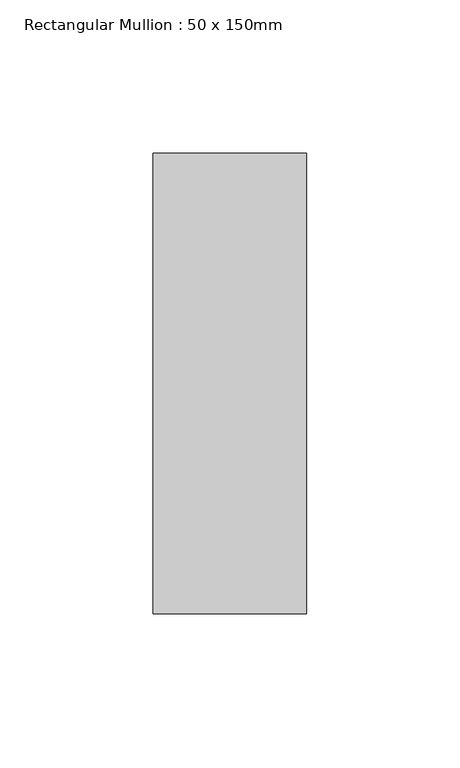
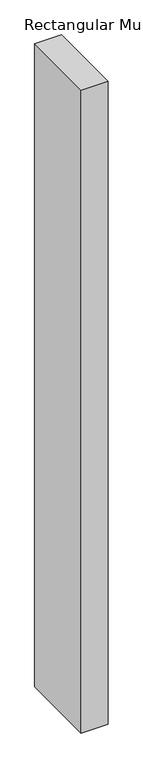
"""IFC4 building model written with IfcOpenShell, lengths in millimetres: member geometry, Rectangular Mullion : 50 x 150mm."""

from ifc_helpers import new_model, si_unit, frame, origin, place, context, project, spatial, polyline, outline, extrude, source, transform, mapped, element, save


def rectangular_mullion_50_x_150mm_673792d4(model_context):
    return source(origin(), model_context, "Body", "SweptSolid", [
        extrude(outline(polyline([(0.0, 75.0), (0.0, -75.0), (-50.0, -75.0), (-50.0, 75.0), (0.0, 75.0)])), frame((0.0, 0.0, -1264.9999999), z_axis=(0.0, 0.0, 1.0), x_axis=(1.0, 0.0, 0.0)), (0.0, 0.0, 1.0), 1264.9999999),
    ])


if __name__ == "__main__":
    model = new_model("IFC4")
    model_context = context("Model", 3, world=origin())
    ifc_project = project(units=[si_unit("LENGTHUNIT", "METRE", prefix="MILLI")], contexts=[model_context])
    site = spatial("IfcSite", under=ifc_project)
    building = spatial("IfcBuilding", under=site)
    placement = place(None, origin())
    rectangular_mullion_50_x_150mm_shape = rectangular_mullion_50_x_150mm_673792d4(model_context)
    element("IfcMember", 1, ObjectType="Rectangular Mullion : 50 x 150mm", at=placement, inside=building, context=model_context, shape_type="MappedRepresentation", body=[
        mapped(rectangular_mullion_50_x_150mm_shape, transform((0.0, 0.0, 0.0), x_axis=(1.0, 0.0, 0.0), y_axis=(0.0, 1.0, 0.0), z_axis=(0.0, 0.0, 1.0))),
    ])
    save(model, "model.ifc")

# Revit data of these elements
# Type "Rectangular Mullion : 50 x 150mm"
#   built-in parameter 1007304 = 0.492126 (stored number, unit not read)
#   built-in parameter 1007301 = 0.082021 (stored number, unit not read)
#   built-in parameter 1007300 = 0.082021 (stored number, unit not read)
# Element 1 (IfcMember, "Rectangular Mullion : 50 x 150mm")
#   Materials on its faces: "Aluminium"
# Materials
#   "Aluminium": class "Metal", colour RGB 247 247 247, transparency 0, Description = "Aluminium 6061", Cost = 0
